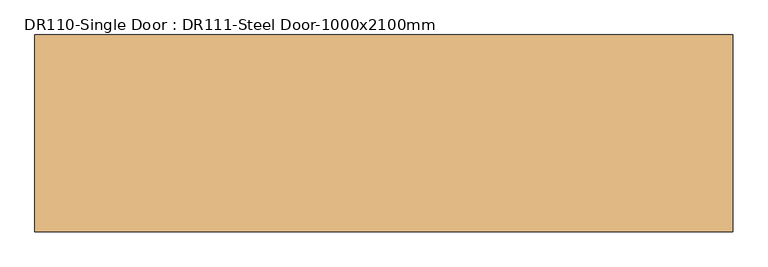
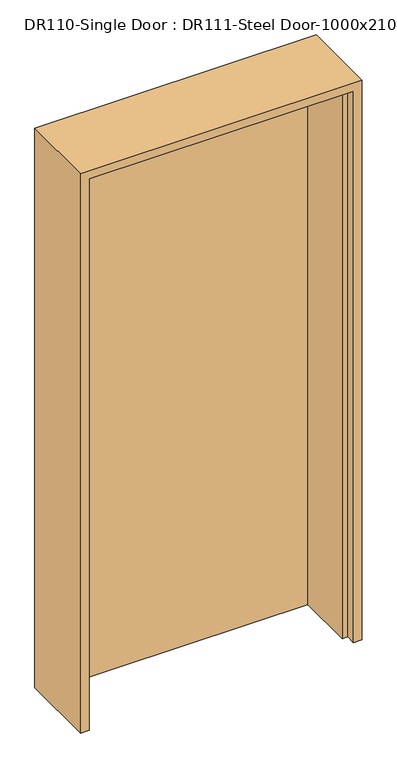
"""IFC4 building model written with IfcOpenShell, lengths in millimetres: door geometry, DR110-Single Door : DR111-Steel Door-1000x2100mm."""

from ifc_helpers import new_model, si_unit, origin, origin_with_axes, place, context, project, spatial, polyline, outline, extrude, faceted_brep, source, transform, mapped, element, save


def dr110_single_door_dr111_steel_door_1000x2100mm_74bb0800(model_context):
    return source(origin(), model_context, "Body", "SolidModel", [
        extrude(outline(polyline([(470.0, 141.0), (470.0, 106.0), (-470.0, 106.0), (-470.0, 141.0), (470.0, 141.0)])), origin_with_axes(), (0.0, 0.0, 1.0), 2070.0),
        faceted_brep([(470.0, 141.0, 0.0), (500.0, 141.0, 0.0), (500.0, -141.0, 0.0), (470.0, -141.0, 0.0), (470.0, -106.0, 0.0), (450.0, -106.0, 0.0), (450.0, 106.0, 0.0), (470.0, 106.0, 0.0), (470.0, 141.0, 2070.0), (-470.0, 141.0, 2070.0), (-470.0, 141.0, 0.0), (-500.0, 141.0, 0.0), (-500.0, 141.0, 2100.0), (500.0, 141.0, 2100.0), (500.0, -141.0, 2100.0), (-500.0, -141.0, 2100.0), (-500.0, -141.0, 0.0), (-470.0, -141.0, 0.0), (-470.0, -141.0, 2070.0), (470.0, -141.0, 2070.0), (470.0, -106.0, 2070.0), (-470.0, -106.0, 2070.0), (-470.0, -106.0, 0.0), (-450.0, -106.0, 0.0), (-450.0, -106.0, 2050.0), (450.0, -106.0, 2050.0), (450.0, 106.0, 2050.0), (-450.0, 106.0, 2050.0), (-450.0, 106.0, 0.0), (-470.0, 106.0, 0.0), (-470.0, 106.0, 2070.0), (470.0, 106.0, 2070.0)], [[[0, 1, 2, 3, 4, 5, 6, 7]], [[1, 0, 8, 9, 10, 11, 12, 13]], [[2, 1, 13, 14]], [[3, 2, 14, 15, 16, 17, 18, 19]], [[4, 3, 19, 20]], [[5, 4, 20, 21, 22, 23, 24, 25]], [[6, 5, 25, 26]], [[7, 6, 26, 27, 28, 29, 30, 31]], [[0, 7, 31, 8]], [[9, 30, 29, 10]], [[10, 29, 28, 23, 22, 17, 16, 11]], [[15, 12, 11, 16]], [[21, 18, 17, 22]], [[27, 24, 23, 28]], [[14, 13, 12, 15]], [[20, 19, 18, 21]], [[26, 25, 24, 27]], [[8, 31, 30, 9]]]),
    ])


if __name__ == "__main__":
    model = new_model("IFC4")
    model_context = context("Model", 3, world=origin())
    ifc_project = project(units=[si_unit("LENGTHUNIT", "METRE", prefix="MILLI")], contexts=[model_context])
    site = spatial("IfcSite", under=ifc_project)
    building = spatial("IfcBuilding", under=site)
    placement = place(None, origin())
    dr110_single_door_dr111_steel_door_1000x2100mm_shape = dr110_single_door_dr111_steel_door_1000x2100mm_74bb0800(model_context)
    element("IfcDoor", 1, ObjectType="DR110-Single Door : DR111-Steel Door-1000x2100mm", at=placement, inside=building, context=model_context, shape_type="MappedRepresentation", body=[
        mapped(dr110_single_door_dr111_steel_door_1000x2100mm_shape, transform((0.0, 0.0, 0.0), x_axis=(1.0, 0.0, 0.0), y_axis=(0.0, 1.0, 0.0), z_axis=(0.0, 0.0, 1.0))),
    ])
    save(model, "model.ifc")

# Revit data of these elements
# Type "DR110-Single Door : DR111-Steel Door-1000x2100mm"
#   Description = "DSDSSD"
#   Type Mark = "SD"
#   Analytic Construction = "<None>"
#   프레임 투영 외부. = 25 mm
#   프레임 투영 내부. = 25 mm
#   프레임 폭 = 75 mm
#   Height = 2100 mm
#   Width = 1000 mm
#   Define Thermal Properties by = 1
#   문 패널 = SD1 문 패널
#   문 프레임 = A04AQ098-00002_Steel Door_non FP_single
#   Function = (empty or 0)
#   Wall Closure = (empty or 0)
# Element 1 (IfcDoor, "DR110-Single Door : DR111-Steel Door-1000x2100mm")
#   Materials on its faces: "A04AQ098-00002_Steel Door_non FP_single", "SD1 문 패널"
# Materials
#   "SD1 문 패널": class "금속", colour RGB 247 247 247, transparency 0, Description = "STEEL DOOR (1000Wx2100H)"
#   "A04AQ098-00002_Steel Door_non FP_single": class "금속", colour RGB 247 247 247, transparency 0, Description = "Steel Door", W00) Work Master Code = "A04AQ098-00002", W01) Work Master_Lv1 = "Finishing Work", W02) Work Master_Lv2 = "Door & Window Work", W03) Work Master_Spec.1 = "Steel Door w/ Steel Frame", W04) Work Master_Spec.2 = "Fire Protective Rating: N/A, Single Door", W05) Work Master_Spec.3 = "w/ Hardware & Accessories", Cost = 0
